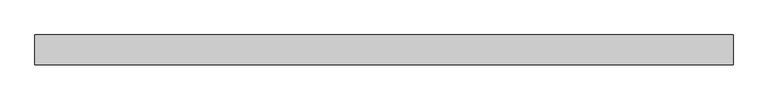
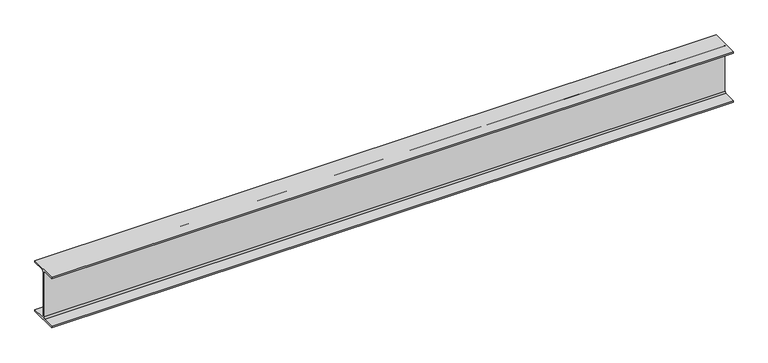
"""IFC4 building model written with IfcOpenShell, lengths in millimetres: beam geometry, Steel Beam_H-KSD3502 : H_SB_ASB_H-250x125x6x9."""

from ifc_helpers import new_model, si_unit, point, frame, frame_2d, origin, place, context, project, spatial, polyline, circle_curve, trimmed, segment, composite_curve, outline, extrude, source, transform, mapped, element, save


def beam_5c55ab62(model_context):
    return source(origin(), model_context, "Body", "SweptSolid", [
        extrude(outline(composite_curve([segment(polyline([(82.5, -141.5), (82.5, -151.7), (-82.5, -151.7), (-82.5, -141.5), (-11.9, -141.5)]), True, "CONTINUOUS"), segment(trimmed(circle_curve(frame_2d((-11.9, -132.6)), 8.9), [point((-11.9, -141.5))], [point((-3.0, -132.6))], True, "CARTESIAN"), True, "CONTINUOUS"), segment(polyline([(-3.0, -132.6), (-3.0, 132.6)]), True, "CONTINUOUS"), segment(trimmed(circle_curve(frame_2d((-11.9, 132.6)), 8.9), [point((-3.0, 132.6))], [point((-11.9, 141.5))], True, "CARTESIAN"), True, "CONTINUOUS"), segment(polyline([(-11.9, 141.5), (-82.5, 141.5), (-82.5, 151.7), (82.5, 151.7), (82.5, 141.5), (11.9, 141.5)]), True, "CONTINUOUS"), segment(trimmed(circle_curve(frame_2d((11.9, 132.6)), 8.9), [point((11.9, 141.5))], [point((3.0, 132.6))], True, "CARTESIAN"), True, "CONTINUOUS"), segment(polyline([(3.0, 132.6), (3.0, -132.6)]), True, "CONTINUOUS"), segment(trimmed(circle_curve(frame_2d((11.9, -132.6)), 8.9), [point((3.0, -132.6))], [point((11.9, -141.5))], True, "CARTESIAN"), True, "CONTINUOUS"), segment(polyline([(11.9, -141.5), (82.5, -141.5)]), True, "CONTINUOUS")], self_intersect=False)), frame((-1830.0829189, 0.0, 0.0), z_axis=(1.0, 0.0, 0.0), x_axis=(0.0, 1.0, 0.0)), (0.0, 0.0, 1.0), 3859.8829189),
    ])


if __name__ == "__main__":
    model = new_model("IFC4")
    model_context = context("Model", 3, world=origin())
    ifc_project = project(units=[si_unit("LENGTHUNIT", "METRE", prefix="MILLI")], contexts=[model_context])
    site = spatial("IfcSite", under=ifc_project)
    building = spatial("IfcBuilding", under=site)
    placement = place(None, origin())
    beam_shape = beam_5c55ab62(model_context)
    element("IfcBeam", 1, ObjectType="Steel Beam_H-KSD3502 : H_SB_ASB_H-250x125x6x9", at=placement, inside=building, context=model_context, shape_type="MappedRepresentation", body=[
        mapped(beam_shape, transform((0.0, 0.0, 0.0), x_axis=(1.0, 0.0, 0.0), y_axis=(0.0, 1.0, 0.0), z_axis=(0.0, 0.0, 1.0))),
    ])
    save(model, "model.ifc")

# Revit data of these elements
# Type "Steel Beam_H-KSD3502 : H_SB_ASB_H-250x125x6x9"
#   Width = 12.5 cm
#   Web Thickness = 0.6 cm
#   Web Fillet = 1.2 cm
#   Warping Constant = 42539.8 cm⁶
#   Torsional Moment of Inertia = 7.8102 cm⁴
#   Torsional Modulus = 1.0 cm³
#   Section Area = 37.66 cm²
#   Plastic Modulus weak axis = 73.1 cm³
#   Plastic Modulus strong axis = 366.0 cm³
#   Perimeter = 0.97 m²/m
#   Nominal Weight = 29.60 kgf/m
#   Moment of Inertia weak axis = 294.00 cm⁴
#   Moment of Inertia strong axis = 4050.00 cm⁴
#   Height = 25.0 cm
#   Flange Thickness = 0.9 cm
#   Elastic Modulus weak axis = 47.0 cm³
#   Elastic Modulus strong axis = 324.0 cm³
#   Centroid Vertical = 12.5 cm
#   Centroid Horizontal = 6.25 cm
#   Length [instance default] = 1.5240 m
#   Structural Material [instance default] = Steel, 45-345
#   Assembly Code = ""
# Element 1 (IfcBeam, "Steel Beam_H-KSD3502 : H_SB_ASB_H-250x125x6x9")
#   Structural Material = none
# Materials
#   "Steel, 45-345": class "Metal", colour RGB 189 187 185, transparency 0, Description = "Steel 345 MPa", Cost = 0
